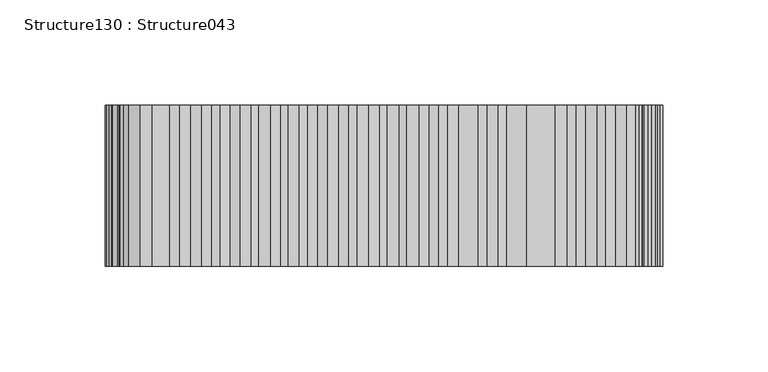
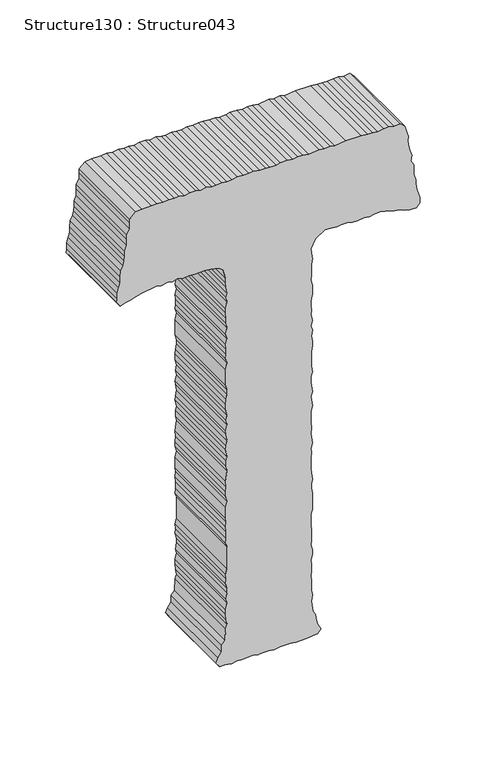
"""IFC4 building model written with IfcOpenShell, lengths in millimetres: proxy geometry, Structure130 : Structure043."""

from ifc_helpers import new_model, si_unit, frame, origin, place, context, project, spatial, polyline, outline, extrude, source, transform, mapped, element, save


def structure130_structure043_2fc135d6(model_context):
    return source(origin(), model_context, "Body", "SweptSolid", [
        extrude(outline(polyline([(3992.8375436, -41987.8855116), (3996.9645864, -41991.9852761), (3996.390138, -41997.2451697), (3997.5486624, -42001.9482654), (3996.9645864, -42006.0480299), (3996.390138, -42011.3079235), (3996.9645864, -42016.0110192), (3996.9645864, -42020.0883193), (3997.5486624, -42025.9499395), (3997.5486624, -42039.4558955), (3996.390138, -42048.8155535), (3997.5486624, -42052.9169226), (3996.9645864, -42058.1752116), (3997.5486624, -42062.2990451), (3996.390138, -42071.6587031), (3997.5486624, -42076.9410611), (3997.5486624, -42081.0408256), (3996.9645864, -42085.7214569), (3997.5486624, -42090.4245527), (3997.5486624, -42096.2621039), (3996.390138, -42099.8066752), (3996.390138, -42105.645831), (3996.9645864, -42109.1663332), (3996.9645864, -42114.4486912), (3997.5486624, -42119.7085848), (3997.5486624, -42123.8083493), (3996.9645864, -42128.511445), (3997.5486624, -42133.769734), (3996.390138, -42138.4503653), (3996.390138, -42143.1534611), (3996.9645864, -42147.2532255), (3996.390138, -42152.5355835), (3996.390138, -42156.0336213), (3997.5486624, -42160.7142527), (3996.390138, -42166.5983373), (3997.5486624, -42170.0963751), (3997.5486624, -42175.3787331), (3996.390138, -42180.0593645), (3997.5486624, -42184.7383912), (3996.9645864, -42188.8622247), (3997.5486624, -42193.5412514), (3996.9645864, -42198.801145), (3997.5486624, -42204.083503), (3996.9645864, -42208.7641343), (3996.9645864, -42216.9652679), (3996.390138, -42222.8252835), (3991.6806238, -42228.1076415), (3988.1633307, -42228.1076415), (3982.8793681, -42228.1076415), (3978.2035506, -42230.4471548), (3974.1214368, -42230.4471548), (3968.2357475, -42230.4471548), (3963.5615346, -42232.2090106), (3958.8776941, -42232.2090106), (3954.7506513, -42232.7882728), (3950.6765605, -42233.3899995), (3946.5511223, -42235.7070484), (3941.2912288, -42236.3087751), (3936.0345445, -42236.3087751), (3931.9058971, -42237.4672995), (3927.2332888, -42238.649893), (3921.9733953, -42238.649893), (3918.4480792, -42239.2291552), (3914.3499193, -42236.3087751), (3916.0909152, -42231.0280217), (3916.6653636, -42227.5283793), (3918.4480792, -42222.8252835), (3919.6066036, -42218.1462568), (3921.3748778, -42204.6852297), (3920.7908018, -42200.5613961), (3921.9733953, -42194.7013805), (3920.7908018, -42190.6000114), (3921.9733953, -42186.5002469), (3920.7908018, -42181.2403534), (3921.3748778, -42176.5372576), (3920.7908018, -42171.2773641), (3921.3748778, -42166.5983373), (3921.3748778, -42163.0762305), (3920.7908018, -42157.2162149), (3919.0321552, -42150.1736057), (3916.6653636, -42146.6514989), (3907.888177, -42144.33445), (3903.7884125, -42144.33445), (3899.1061766, -42143.7327233), (3893.822214, -42143.1534611), (3890.320967, -42143.7327233), (3885.6210804, -42143.1534611), (3879.7610648, -42144.33445), (3876.263027, -42144.33445), (3870.9790644, -42143.7327233), (3866.3032469, -42143.7327233), (3861.6178018, -42143.1534611), (3856.3161885, -42144.33445), (3851.6612309, -42143.1534611), (3846.9757858, -42144.33445), (3842.2758992, -42143.7327233), (3837.6000817, -42143.7327233), (3833.4730389, -42144.33445), (3829.374879, -42143.1534611), (3823.5341187, -42144.33445), (3809.4729695, -42144.33445), (3804.7730829, -42143.1534611), (3800.6717138, -42143.1534611), (3795.960595, -42143.7327233), (3791.8865042, -42144.33445), (3786.6298199, -42144.33445), (3781.3282066, -42143.1534611), (3776.6427615, -42143.7327233), (3772.5606477, -42143.1534611), (3767.2590344, -42144.33445), (3763.759392, -42143.7327233), (3757.8753073, -42143.1534611), (3753.2171405, -42143.7327233), (3749.701452, -42144.33445), (3743.2332913, -42143.1534611), (3739.7416719, -42143.7327233), (3734.47536, -42143.7327233), (3730.3563402, -42143.1534611), (3720.9726131, -42144.33445), (3715.7143242, -42143.7327233), (3711.0304837, -42144.33445), (3706.9130685, -42144.33445), (3702.229228, -42143.1534611), (3696.9709391, -42144.33445), (3687.0127636, -42144.33445), (3683.4858429, -42143.7327233), (3678.81163, -42144.33445), (3674.1277895, -42143.7327233), (3668.2437048, -42143.7327233), (3663.5598643, -42144.33445), (3660.0682449, -42143.1534611), (3640.114988, -42143.1534611), (3635.4407751, -42144.33445), (3630.7392839, -42143.7327233), (3626.6571701, -42144.33445), (3621.9813526, -42143.1534611), (3617.8559144, -42143.1534611), (3612.0135494, -42143.7327233), (3608.4705827, -42143.1534611), (3602.6298224, -42144.33445), (3598.5284533, -42144.33445), (3593.2541183, -42143.7327233), (3588.5702778, -42143.1534611), (3585.0706354, -42144.33445), (3574.5107332, -42144.9137122), (3570.9854171, -42147.8324878), (3565.1254015, -42147.8324878), (3560.441561, -42150.7753324), (3556.3417965, -42152.5355835), (3551.6675836, -42149.5943435), (3552.242032, -42144.9137122), (3551.0658569, -42139.0296275), (3552.242032, -42134.3506008), (3551.6675836, -42130.2716962), (3552.242032, -42124.9893382), (3552.242032, -42120.3103115), (3551.0658569, -42116.1864779), (3551.6675836, -42112.0867134), (3551.6675836, -42106.8268199), (3551.0658569, -42102.1237241), (3551.6675836, -42096.8638306), (3551.6675836, -42087.4817081), (3551.0658569, -42082.8026814), (3551.0658569, -42079.2805745), (3551.6675836, -42073.4189543), (3552.242032, -42068.7399276), (3552.242032, -42064.0368318), (3555.7416744, -42061.1180562), (3561.6257591, -42064.0368318), (3565.1254015, -42065.2178207), (3570.9854171, -42065.7970829), (3574.5107332, -42068.1606653), (3583.8864372, -42069.3191898), (3589.7544759, -42068.7399276), (3594.4286888, -42069.3191898), (3602.6298224, -42069.3191898), (3607.8961343, -42069.9209165), (3612.5976255, -42069.3191898), (3617.2718384, -42069.3191898), (3622.555801, -42069.9209165), (3627.2396415, -42068.7399276), (3631.3410106, -42068.7399276), (3636.0408972, -42069.9209165), (3640.7167147, -42069.3191898), (3649.5003197, -42069.3191898), (3655.3587307, -42069.9209165), (3664.7440624, -42069.9209165), (3668.8261762, -42068.7399276), (3683.4858429, -42068.7399276), (3688.1873341, -42069.3191898), (3692.2710525, -42069.3191898), (3696.3884676, -42068.7399276), (3702.229228, -42069.3191898), (3706.3289925, -42069.9209165), (3716.2887726, -42069.9209165), (3720.9726131, -42069.3191898), (3725.0996559, -42069.9209165), (3729.7738688, -42068.7399276), (3735.0578314, -42069.3191898), (3738.5574738, -42069.9209165), (3744.4158848, -42069.3191898), (3749.117376, -42069.9209165), (3759.0595054, -42069.9209165), (3763.759392, -42068.7399276), (3773.11905, -42069.9209165), (3776.6427615, -42068.7399276), (3786.0280932, -42069.9209165), (3791.3056374, -42069.9209165), (3795.4037973, -42068.7399276), (3800.6717138, -42069.3191898), (3814.148787, -42069.3191898), (3819.4150989, -42068.7399276), (3823.5341187, -42068.7399276), (3828.2163546, -42069.3191898), (3834.0474873, -42068.7399276), (3837.6000817, -42069.9209165), (3842.8583706, -42068.7399276), (3848.1166595, -42069.9209165), (3851.6612309, -42069.3191898), (3857.5019912, -42069.9209165), (3861.0192843, -42069.9209165), (3866.8776953, -42068.7399276), (3875.0772243, -42068.7399276), (3879.7610648, -42069.9209165), (3885.6210804, -42069.3191898), (3894.4030808, -42069.3191898), (3899.1061766, -42068.7399276), (3904.3901392, -42069.3191898), (3909.0627475, -42069.9209165), (3916.6653636, -42065.7970829), (3921.9733953, -42057.5959493), (3921.9733953, -42052.9169226), (3921.3748778, -42047.0553024), (3921.9733953, -42043.5331955), (3921.9733953, -42038.2749066), (3920.7908018, -42033.5718108), (3920.7908018, -42029.4704417), (3921.3748778, -42023.6328906), (3920.7908018, -42018.9297948), (3921.3748778, -42014.8284257), (3921.9733953, -42009.5701368), (3919.6066036, -42000.7672765), (3918.4480792, -41997.2451697), (3917.8479571, -41992.5645383), (3916.0909152, -41988.4647739), (3914.9307861, -41983.7841425), (3914.3499193, -41977.9225223), (3917.8479571, -41974.9812823), (3923.1319197, -41974.9812823), (3927.2332888, -41976.1622712), (3931.3346579, -41977.3432601), (3937.1930689, -41978.5033892), (3940.718385, -41978.5033892), (3945.9766739, -41980.2636403), (3951.2606365, -41980.2636403), (3954.7506513, -41980.2636403), (3959.4617701, -41982.6031536), (3964.1343784, -41982.001427), (3969.418341, -41983.7841425), (3972.9372387, -41984.3634048), (3978.2035506, -41985.5443937), (3982.8793681, -41984.942667), (3987.0048063, -41986.1252605), (3992.8375436, -41987.8855116)])), frame((0.0, 247945.1599557, 0.0), z_axis=(0.0, 1.0, 0.0), x_axis=(0.0, 0.0, 1.0)), (0.0, 0.0, 1.0), 76.2),
    ])


if __name__ == "__main__":
    model = new_model("IFC4")
    model_context = context("Model", 3, world=origin())
    ifc_project = project(units=[si_unit("LENGTHUNIT", "METRE", prefix="MILLI")], contexts=[model_context])
    site = spatial("IfcSite", under=ifc_project)
    building = spatial("IfcBuilding", under=site)
    placement = place(None, origin())
    structure130_structure043_shape = structure130_structure043_2fc135d6(model_context)
    element("IfcBuildingElementProxy", 1, Name="Structure130 : Structure043", ObjectType="Structure130 : Structure043", at=placement, inside=building, context=model_context, shape_type="MappedRepresentation", body=[
        mapped(structure130_structure043_shape, transform((0.0, 0.0, 0.0), x_axis=(1.0, 0.0, 0.0), y_axis=(0.0, 1.0, 0.0), z_axis=(0.0, 0.0, 1.0))),
    ])
    save(model, "model.ifc")

# Revit data of these elements
# Type "Structure130 : Structure043"
#   NameOverride = "Structure043"
# Element 1 (IfcBuildingElementProxy, "Structure130 : Structure043")
#   Materials on its faces: "BRUSHED ALUM. LETTERING"
# Materials
#   "BRUSHED ALUM. LETTERING": class "Unassigned", colour RGB 169 181 186, transparency 0, Cost = 0
